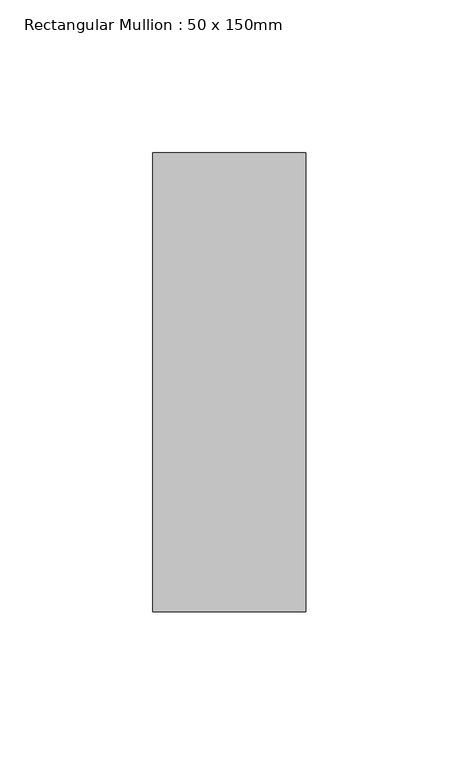
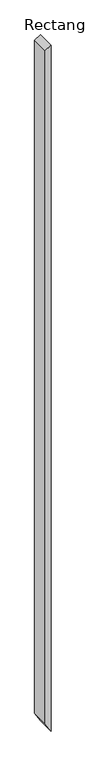
"""IFC4 building model written with IfcOpenShell, lengths in millimetres: member geometry, Rectangular Mullion : 50 x 150mm."""

from ifc_helpers import new_model, si_unit, frame, origin, place, context, project, spatial, polyline, outline, extrude, source, transform, mapped, element, save


def rectangular_mullion_50_x_150mm_9d0fdde0(model_context):
    return source(origin(), model_context, "Body", "SweptSolid", [
        extrude(outline(polyline([(0.0, 0.0), (-29.8865247, -50.0), (-5931.3660368, -50.0), (-6015.015776, 0.0), (0.0, 0.0)])), frame((0.0, -75.0, 0.0), z_axis=(0.0, 1.0, 0.0), x_axis=(0.0, 0.0, 1.0)), (0.0, 0.0, 1.0), 150.0),
    ])


if __name__ == "__main__":
    model = new_model("IFC4")
    model_context = context("Model", 3, world=origin())
    ifc_project = project(units=[si_unit("LENGTHUNIT", "METRE", prefix="MILLI")], contexts=[model_context])
    site = spatial("IfcSite", under=ifc_project)
    building = spatial("IfcBuilding", under=site)
    placement = place(None, origin())
    rectangular_mullion_50_x_150mm_shape = rectangular_mullion_50_x_150mm_9d0fdde0(model_context)
    element("IfcMember", 1, ObjectType="Rectangular Mullion : 50 x 150mm", at=placement, inside=building, context=model_context, shape_type="MappedRepresentation", body=[
        mapped(rectangular_mullion_50_x_150mm_shape, transform((0.0, 0.0, 0.0), x_axis=(1.0, 0.0, 0.0), y_axis=(0.0, 1.0, 0.0), z_axis=(0.0, 0.0, 1.0))),
    ])
    save(model, "model.ifc")

# Revit data of these elements
# Type "Rectangular Mullion : 50 x 150mm"
#   built-in parameter 1007304 = 0.492126 (stored number, unit not read)
#   built-in parameter 1007301 = 0.082021 (stored number, unit not read)
#   built-in parameter 1007300 = 0.082021 (stored number, unit not read)
# Element 1 (IfcMember, "Rectangular Mullion : 50 x 150mm")
#   Materials on its faces: "Metal - Aluminium"
# Materials
#   "Metal - Aluminium": class "Metal", colour RGB 247 247 247, transparency 0
